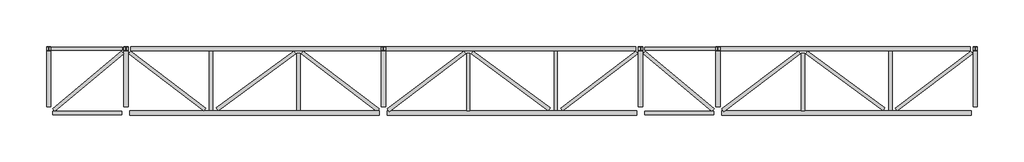
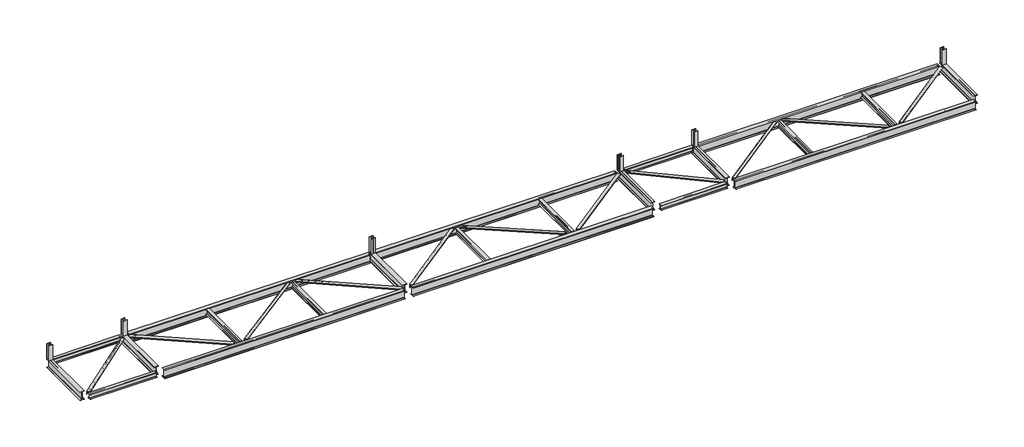
# One storey: 22 beams, 11 members, 6 columns.
"""IFC4 building model written with IfcOpenShell, lengths in millimetres."""

import ifcopenshell
import ifcopenshell.guid

model = None  # the IFC model being written
_history = None  # IfcOwnerHistory: only IFC2X3 demands one
_inside = {}  # id of a spatial element -> (the spatial element, [elements in it])
_under = {}  # id of a project, library or spatial element -> (it, [spatial elements below it])
_declared = {}  # id of a project -> (the project, [libraries it declares])
_typed = {}  # id of a type object -> (the type object, [elements of that type])
_made_of = {}  # id of a material, layer set ... -> (it, [elements and type objects made of it])


def new_model(schema):
    """Start an empty IFC model of exactly this schema.

    Asked for "IFC4X3", IfcOpenShell would pick the latest addendum, in which some entities
    have other attributes; the version numbers below select the first issue.
    IFC2X3 requires an IfcOwnerHistory on every rooted entity: one is made here for all.
    """
    global model, _history
    if schema == "IFC4X3":
        model = ifcopenshell.file(schema_version=(4, 3, 0, 0))
    else:
        model = ifcopenshell.file(schema=schema)
    _inside.clear()
    _under.clear()
    _declared.clear()
    _typed.clear()
    _made_of.clear()
    _history = None
    if model.schema == "IFC2X3":
        org = make("IfcOrganization", Name="unknown")
        user = make(
            "IfcPersonAndOrganization",
            ThePerson=make("IfcPerson", FamilyName="unknown"),
            TheOrganization=org,
        )
        app = make(
            "IfcApplication",
            ApplicationDeveloper=org,
            Version="unknown",
            ApplicationFullName="unknown",
            ApplicationIdentifier="unknown",
        )
        _history = make(
            "IfcOwnerHistory",
            OwningUser=user,
            OwningApplication=app,
            ChangeAction="ADDED",
            CreationDate=0,
        )
    return model


def make(cls, **values):
    """One entity of the class cls with the attributes given. An attribute that is None is left unset."""
    return model.create_entity(
        cls, **{name: value for name, value in values.items() if value is not None}
    )


def rooted(cls, **values):
    """An entity with a GlobalId (a new one), such as an element, a storey or a relation."""
    return make(cls, GlobalId=ifcopenshell.guid.new(), OwnerHistory=_history, **values)


def si_unit(unit_type, name, prefix=None):
    """IfcSIUnit, for example si_unit("LENGTHUNIT", "METRE", prefix="MILLI")."""
    return make("IfcSIUnit", UnitType=unit_type, Prefix=prefix, Name=name)


def assignment(units):
    """IfcUnitAssignment: the units of a project."""
    return None if units is None else make("IfcUnitAssignment", Units=units)


def point(xyz):
    """IfcCartesianPoint."""
    return None if xyz is None else make("IfcCartesianPoint", Coordinates=xyz)


def direction(xyz):
    """IfcDirection."""
    return None if xyz is None else make("IfcDirection", DirectionRatios=xyz)


def frame(location, z_axis=None, x_axis=None):
    """IfcAxis2Placement3D, a coordinate frame: its origin and axes. An axis left out is left unset."""
    return make(
        "IfcAxis2Placement3D",
        Location=point(location),
        Axis=direction(z_axis),
        RefDirection=direction(x_axis),
    )


def frame_2d(location, x_axis=None):
    """IfcAxis2Placement2D, a coordinate frame in the plane: its origin and x axis."""
    return make(
        "IfcAxis2Placement2D", Location=point(location), RefDirection=direction(x_axis)
    )


def origin():
    """The frame at (0, 0, 0) with its axes left unset."""
    return frame((0.0, 0.0, 0.0))


def place(relative_to, where):
    """IfcLocalPlacement: puts the frame where relative to a parent placement (None: the world)."""
    return make(
        "IfcLocalPlacement", PlacementRelTo=relative_to, RelativePlacement=where
    )


def context(
    kind, dimensions, precision=None, world=None, true_north=None, identifier=None
):
    """IfcGeometricRepresentationContext, for example the 3D "Model" context."""
    return make(
        "IfcGeometricRepresentationContext",
        ContextIdentifier=identifier,
        ContextType=kind,
        CoordinateSpaceDimension=dimensions,
        Precision=precision,
        WorldCoordinateSystem=world,
        TrueNorth=true_north,
    )


def project(units=None, contexts=None):
    """IfcProject with its units and contexts."""
    return rooted(
        "IfcProject",
        Name="project",
        RepresentationContexts=contexts,
        UnitsInContext=assignment(units),
    )


def spatial(cls, under=None, at=None, **own):
    """A site, building, storey or space (cls), placed at a placement, below another one or the project."""
    s = rooted(cls, ObjectPlacement=at, **own)
    if under is not None:
        _under.setdefault(under.id(), (under, []))[1].append(s)
    return s


def polyline(points):
    """IfcPolyline through the points."""
    return make("IfcPolyline", Points=[point(p) for p in points])


def circle_curve(where, radius):
    """IfcCircle in the frame where."""
    return make("IfcCircle", Position=where, Radius=radius)


def trimmed(basis, trim1, trim2, sense, master):
    """IfcTrimmedCurve: the piece of a basis curve between two trims."""
    return make(
        "IfcTrimmedCurve",
        BasisCurve=basis,
        Trim1=trim1,
        Trim2=trim2,
        SenseAgreement=sense,
        MasterRepresentation=master,
    )


def segment(curve, same_sense, transition):
    """IfcCompositeCurveSegment."""
    return make(
        "IfcCompositeCurveSegment",
        Transition=transition,
        SameSense=same_sense,
        ParentCurve=curve,
    )


def composite_curve(segments, self_intersect=None):
    """IfcCompositeCurve: segments joined end to end."""
    return make("IfcCompositeCurve", Segments=segments, SelfIntersect=self_intersect)


def outline(outer, holes=None, kind="AREA"):
    """IfcArbitraryClosedProfileDef: a profile drawn as a closed curve; with holes, ...WithVoids."""
    if holes is None:
        return make("IfcArbitraryClosedProfileDef", ProfileType=kind, OuterCurve=outer)
    return make(
        "IfcArbitraryProfileDefWithVoids",
        ProfileType=kind,
        OuterCurve=outer,
        InnerCurves=holes,
    )


def extrude(swept, where, along, depth):
    """IfcExtrudedAreaSolid: the profile swept, set in the frame where, extruded along a direction by depth."""
    return make(
        "IfcExtrudedAreaSolid",
        SweptArea=swept,
        Position=where,
        ExtrudedDirection=direction(along),
        Depth=depth,
    )


def shape(context_of_items, identifier, shape_type, items):
    """IfcShapeRepresentation: the items that make up one representation, for example the "Body"."""
    return make(
        "IfcShapeRepresentation",
        ContextOfItems=context_of_items,
        RepresentationIdentifier=identifier,
        RepresentationType=shape_type,
        Items=items,
    )


def source(mapping_origin, context_of_items, identifier, shape_type, items):
    """IfcRepresentationMap: a shape defined once, which mapped items show again and again."""
    return make(
        "IfcRepresentationMap",
        MappingOrigin=mapping_origin,
        MappedRepresentation=shape(context_of_items, identifier, shape_type, items),
    )


def transform(
    local_origin,
    x_axis=None,
    y_axis=None,
    z_axis=None,
    scale=None,
    scale2=None,
    scale3=None,
    uniform=True,
):
    """IfcCartesianTransformationOperator3D, or its non-uniform kind. x_axis, y_axis, z_axis: its Axis1, 2, 3."""
    if uniform:
        return make(
            "IfcCartesianTransformationOperator3D",
            Axis1=direction(x_axis),
            Axis2=direction(y_axis),
            LocalOrigin=point(local_origin),
            Scale=scale,
            Axis3=direction(z_axis),
        )
    return make(
        "IfcCartesianTransformationOperator3DnonUniform",
        Axis1=direction(x_axis),
        Axis2=direction(y_axis),
        LocalOrigin=point(local_origin),
        Scale=scale,
        Axis3=direction(z_axis),
        Scale2=scale2,
        Scale3=scale3,
    )


def mapped(mapping_source, mapping_target):
    """IfcMappedItem: shows the shape of a source again, moved by a transform."""
    return make(
        "IfcMappedItem", MappingSource=mapping_source, MappingTarget=mapping_target
    )


def made_of(thing, what):
    """Note that an element or type object is made of a material, layer set ...; save() writes the relation."""
    if what is not None:
        _made_of.setdefault(what.id(), (what, []))[1].append(thing)
    return thing


def element(
    cls,
    number,
    at=None,
    inside=None,
    cuts=None,
    type_object=None,
    material=None,
    context=None,
    identifier="Body",
    shape_type=None,
    held_by="IfcProductDefinitionShape",
    body=None,
    shapes=None,
    **own,
):
    """One element of the class cls, such as IfcWall. Its Tag is "e" and its number.

    at: its placement. inside: the storey or other place that contains it. cuts: it is an
    opening in that element (IfcRelVoidsElement). A single representation is given by context,
    identifier, shape_type and body (its items); several are given by shapes. held_by: the class
    of the entity that holds the representations. save() writes the other relations.
    """
    e = rooted(cls, Tag="e%d" % number, ObjectPlacement=at, **own)
    if body is not None:
        shapes = [shape(context, identifier, shape_type, body)]
    if shapes is not None:
        e.Representation = make(held_by, Representations=shapes)
    if inside is not None:
        _inside.setdefault(inside.id(), (inside, []))[1].append(e)
    if cuts is not None:
        rooted(
            "IfcRelVoidsElement", RelatingBuildingElement=cuts, RelatedOpeningElement=e
        )
    if type_object is not None:
        _typed.setdefault(type_object.id(), (type_object, []))[1].append(e)
    return made_of(e, material)


def aggregate(whole, parts):
    """IfcRelAggregates: a whole, such as a stair, and the parts it consists of."""
    return rooted("IfcRelAggregates", RelatingObject=whole, RelatedObjects=parts)


def save(model, path):
    """Write the relations noted so far, then the file.

    IfcRelAggregates (storeys below a building ...), IfcRelContainedInSpatialStructure (elements
    in a storey), IfcRelDefinesByType, IfcRelAssociatesMaterial and IfcRelDeclares: one each for
    every whole, place, type object, material and project.
    """
    for whole, parts in _under.values():
        aggregate(whole, parts)
    for where, things in _inside.values():
        rooted(
            "IfcRelContainedInSpatialStructure",
            RelatedElements=things,
            RelatingStructure=where,
        )
    for kind, things in _typed.values():
        rooted("IfcRelDefinesByType", RelatedObjects=things, RelatingType=kind)
    for what, things in _made_of.values():
        rooted("IfcRelAssociatesMaterial", RelatedObjects=things, RelatingMaterial=what)
    for by, libraries in _declared.values():
        rooted("IfcRelDeclares", RelatingContext=by, RelatedDefinitions=libraries)
    model.write(path)


def steel_framing_w_astm_a6m_f33feb28(model_context):
    return source(origin(), model_context, "Body", "SweptSolid", [
        extrude(outline(composite_curve([segment(polyline([(67.0, -94.8), (67.0, -105.0), (-67.0, -105.0), (-67.0, -94.8), (-10.775, -94.8)]), True, "CONTINUOUS"), segment(trimmed(circle_curve(frame_2d((-10.775, -87.2)), 7.6), [point((-10.775, -94.8))], [point((-3.175, -87.2))], True, "CARTESIAN"), True, "CONTINUOUS"), segment(polyline([(-3.175, -87.2), (-3.175, 87.2)]), True, "CONTINUOUS"), segment(trimmed(circle_curve(frame_2d((-10.775, 87.2)), 7.6), [point((-3.175, 87.2))], [point((-10.775, 94.8))], True, "CARTESIAN"), True, "CONTINUOUS"), segment(polyline([(-10.775, 94.8), (-67.0, 94.8), (-67.0, 105.0), (67.0, 105.0), (67.0, 94.8), (10.775, 94.8)]), True, "CONTINUOUS"), segment(trimmed(circle_curve(frame_2d((10.775, 87.2)), 7.6), [point((10.775, 94.8))], [point((3.175, 87.2))], True, "CARTESIAN"), True, "CONTINUOUS"), segment(polyline([(3.175, 87.2), (3.175, -87.2)]), True, "CONTINUOUS"), segment(trimmed(circle_curve(frame_2d((10.775, -87.2)), 7.6), [point((3.175, -87.2))], [point((10.775, -94.8))], True, "CARTESIAN"), True, "CONTINUOUS"), segment(polyline([(10.775, -94.8), (67.0, -94.8)]), True, "CONTINUOUS")], self_intersect=False)), frame((-1346.3, 0.0, 0.0), z_axis=(1.0, 0.0, 0.0), x_axis=(0.0, 1.0, 0.0)), (0.0, 0.0, 1.0), 2692.6),
    ])


def steel_framing_w_astm_a6m_aee8f6e1(model_context):
    return source(origin(), model_context, "Body", "SweptSolid", [
        extrude(outline(composite_curve([segment(polyline([(85.5, -166.4), (85.5, -178.0), (-85.5, -178.0), (-85.5, -166.4), (-13.72, -166.4)]), True, "CONTINUOUS"), segment(trimmed(circle_curve(frame_2d((-13.72, -156.3)), 10.1), [point((-13.72, -166.4))], [point((-3.62, -156.3))], True, "CARTESIAN"), True, "CONTINUOUS"), segment(polyline([(-3.62, -156.3), (-3.62, 156.3)]), True, "CONTINUOUS"), segment(trimmed(circle_curve(frame_2d((-13.72, 156.3)), 10.1), [point((-3.62, 156.3))], [point((-13.72, 166.4))], True, "CARTESIAN"), True, "CONTINUOUS"), segment(polyline([(-13.72, 166.4), (-85.5, 166.4), (-85.5, 178.0), (85.5, 178.0), (85.5, 166.4), (13.72, 166.4)]), True, "CONTINUOUS"), segment(trimmed(circle_curve(frame_2d((13.72, 156.3)), 10.1), [point((13.72, 166.4))], [point((3.62, 156.3))], True, "CARTESIAN"), True, "CONTINUOUS"), segment(polyline([(3.62, 156.3), (3.62, -156.3)]), True, "CONTINUOUS"), segment(trimmed(circle_curve(frame_2d((13.72, -156.3)), 10.1), [point((3.62, -156.3))], [point((13.72, -166.4))], True, "CARTESIAN"), True, "CONTINUOUS"), segment(polyline([(13.72, -166.4), (85.5, -166.4)]), True, "CONTINUOUS")], self_intersect=False)), frame((-4846.3, 0.0, 0.0), z_axis=(1.0, 0.0, 0.0), x_axis=(0.0, 1.0, 0.0)), (0.0, 0.0, 1.0), 9692.6),
    ])


def steel_framing_w_astm_a6m_761fb5d6(model_context):
    return source(origin(), model_context, "Body", "SweptSolid", [
        extrude(outline(composite_curve([segment(polyline([(85.5, -166.4), (85.5, -178.0), (-85.5, -178.0), (-85.5, -166.4), (-13.72, -166.4)]), True, "CONTINUOUS"), segment(trimmed(circle_curve(frame_2d((-13.72, -156.3)), 10.1), [point((-13.72, -166.4))], [point((-3.62, -156.3))], True, "CARTESIAN"), True, "CONTINUOUS"), segment(polyline([(-3.62, -156.3), (-3.62, 156.3)]), True, "CONTINUOUS"), segment(trimmed(circle_curve(frame_2d((-13.72, 156.3)), 10.1), [point((-3.62, 156.3))], [point((-13.72, 166.4))], True, "CARTESIAN"), True, "CONTINUOUS"), segment(polyline([(-13.72, 166.4), (-85.5, 166.4), (-85.5, 178.0), (85.5, 178.0), (85.5, 166.4), (13.72, 166.4)]), True, "CONTINUOUS"), segment(trimmed(circle_curve(frame_2d((13.72, 156.3)), 10.1), [point((13.72, 166.4))], [point((3.62, 156.3))], True, "CARTESIAN"), True, "CONTINUOUS"), segment(polyline([(3.62, 156.3), (3.62, -156.3)]), True, "CONTINUOUS"), segment(trimmed(circle_curve(frame_2d((13.72, -156.3)), 10.1), [point((3.62, -156.3))], [point((13.72, -166.4))], True, "CARTESIAN"), True, "CONTINUOUS"), segment(polyline([(13.72, -166.4), (85.5, -166.4)]), True, "CONTINUOUS")], self_intersect=False)), frame((-1003.8, 0.0, 0.0), z_axis=(1.0, 0.0, 0.0), x_axis=(0.0, 1.0, 0.0)), (0.0, 0.0, 1.0), 2339.3),
    ])


def steel_framing_w_astm_a6m_44bd27a9(model_context):
    return source(origin(), model_context, "Body", "SweptSolid", [
        extrude(outline(composite_curve([segment(polyline([(85.5, -166.4), (85.5, -178.0), (-85.5, -178.0), (-85.5, -166.4), (-13.72, -166.4)]), True, "CONTINUOUS"), segment(trimmed(circle_curve(frame_2d((-13.72, -156.3)), 10.1), [point((-13.72, -166.4))], [point((-3.62, -156.3))], True, "CARTESIAN"), True, "CONTINUOUS"), segment(polyline([(-3.62, -156.3), (-3.62, 156.3)]), True, "CONTINUOUS"), segment(trimmed(circle_curve(frame_2d((-13.72, 156.3)), 10.1), [point((-3.62, 156.3))], [point((-13.72, 166.4))], True, "CARTESIAN"), True, "CONTINUOUS"), segment(polyline([(-13.72, 166.4), (-85.5, 166.4), (-85.5, 178.0), (85.5, 178.0), (85.5, 166.4), (13.72, 166.4)]), True, "CONTINUOUS"), segment(trimmed(circle_curve(frame_2d((13.72, 156.3)), 10.1), [point((13.72, 166.4))], [point((3.62, 156.3))], True, "CARTESIAN"), True, "CONTINUOUS"), segment(polyline([(3.62, 156.3), (3.62, -156.3)]), True, "CONTINUOUS"), segment(trimmed(circle_curve(frame_2d((13.72, -156.3)), 10.1), [point((3.62, -156.3))], [point((13.72, -166.4))], True, "CARTESIAN"), True, "CONTINUOUS"), segment(polyline([(13.72, -166.4), (85.5, -166.4)]), True, "CONTINUOUS")], self_intersect=False)), frame((-1003.8, 0.0, 0.0), z_axis=(1.0, 0.0, 0.0), x_axis=(0.0, 1.0, 0.0)), (0.0, 0.0, 1.0), 2320.8),
    ])


def steel_framing_w_astm_a6m_88cf460a(model_context):
    return source(origin(), model_context, "Body", "SweptSolid", [
        extrude(outline(composite_curve([segment(polyline([(67.0, -94.8), (67.0, -105.0), (-67.0, -105.0), (-67.0, -94.8), (-10.775, -94.8)]), True, "CONTINUOUS"), segment(trimmed(circle_curve(frame_2d((-10.775, -87.2)), 7.6), [point((-10.775, -94.8))], [point((-3.175, -87.2))], True, "CARTESIAN"), True, "CONTINUOUS"), segment(polyline([(-3.175, -87.2), (-3.175, 87.2)]), True, "CONTINUOUS"), segment(trimmed(circle_curve(frame_2d((-10.775, 87.2)), 7.6), [point((-3.175, 87.2))], [point((-10.775, 94.8))], True, "CARTESIAN"), True, "CONTINUOUS"), segment(polyline([(-10.775, 94.8), (-67.0, 94.8), (-67.0, 105.0), (67.0, 105.0), (67.0, 94.8), (10.775, 94.8)]), True, "CONTINUOUS"), segment(trimmed(circle_curve(frame_2d((10.775, 87.2)), 7.6), [point((10.775, 94.8))], [point((3.175, 87.2))], True, "CARTESIAN"), True, "CONTINUOUS"), segment(polyline([(3.175, 87.2), (3.175, -87.2)]), True, "CONTINUOUS"), segment(trimmed(circle_curve(frame_2d((10.775, -87.2)), 7.6), [point((3.175, -87.2))], [point((10.775, -94.8))], True, "CARTESIAN"), True, "CONTINUOUS"), segment(polyline([(10.775, -94.8), (67.0, -94.8)]), True, "CONTINUOUS")], self_intersect=False)), frame((-1401.8, 0.0, 0.0), z_axis=(1.0, 0.0, 0.0), x_axis=(0.0, 1.0, 0.0)), (0.0, 0.0, 1.0), 2751.8),
    ])


def steel_framing_w_astm_a6m_bf6e2db3(model_context):
    return source(origin(), model_context, "Body", "SweptSolid", [
        extrude(outline(composite_curve([segment(polyline([(85.5, -166.4), (85.5, -178.0), (-85.5, -178.0), (-85.5, -166.4), (-13.72, -166.4)]), True, "CONTINUOUS"), segment(trimmed(circle_curve(frame_2d((-13.72, -156.3)), 10.1), [point((-13.72, -166.4))], [point((-3.62, -156.3))], True, "CARTESIAN"), True, "CONTINUOUS"), segment(polyline([(-3.62, -156.3), (-3.62, 156.3)]), True, "CONTINUOUS"), segment(trimmed(circle_curve(frame_2d((-13.72, 156.3)), 10.1), [point((-3.62, 156.3))], [point((-13.72, 166.4))], True, "CARTESIAN"), True, "CONTINUOUS"), segment(polyline([(-13.72, 166.4), (-85.5, 166.4), (-85.5, 178.0), (85.5, 178.0), (85.5, 166.4), (13.72, 166.4)]), True, "CONTINUOUS"), segment(trimmed(circle_curve(frame_2d((13.72, 156.3)), 10.1), [point((13.72, 166.4))], [point((3.62, 156.3))], True, "CARTESIAN"), True, "CONTINUOUS"), segment(polyline([(3.62, 156.3), (3.62, -156.3)]), True, "CONTINUOUS"), segment(trimmed(circle_curve(frame_2d((13.72, -156.3)), 10.1), [point((3.62, -156.3))], [point((13.72, -166.4))], True, "CARTESIAN"), True, "CONTINUOUS"), segment(polyline([(13.72, -166.4), (85.5, -166.4)]), True, "CONTINUOUS")], self_intersect=False)), frame((-4814.1, 0.0, 0.0), z_axis=(1.0, 0.0, 0.0), x_axis=(0.0, 1.0, 0.0)), (0.0, 0.0, 1.0), 9715.9),
    ])


def steel_framing_w_astm_a6m_6b735529(model_context):
    return source(origin(), model_context, "Body", "SweptSolid", [
        extrude(outline(composite_curve([segment(polyline([(67.0, -94.8), (67.0, -105.0), (-67.0, -105.0), (-67.0, -94.8), (-10.775, -94.8)]), True, "CONTINUOUS"), segment(trimmed(circle_curve(frame_2d((-10.775, -87.2)), 7.6), [point((-10.775, -94.8))], [point((-3.175, -87.2))], True, "CARTESIAN"), True, "CONTINUOUS"), segment(polyline([(-3.175, -87.2), (-3.175, 87.2)]), True, "CONTINUOUS"), segment(trimmed(circle_curve(frame_2d((-10.775, 87.2)), 7.6), [point((-3.175, 87.2))], [point((-10.775, 94.8))], True, "CARTESIAN"), True, "CONTINUOUS"), segment(polyline([(-10.775, 94.8), (-67.0, 94.8), (-67.0, 105.0), (67.0, 105.0), (67.0, 94.8), (10.775, 94.8)]), True, "CONTINUOUS"), segment(trimmed(circle_curve(frame_2d((10.775, 87.2)), 7.6), [point((10.775, 94.8))], [point((3.175, 87.2))], True, "CARTESIAN"), True, "CONTINUOUS"), segment(polyline([(3.175, 87.2), (3.175, -87.2)]), True, "CONTINUOUS"), segment(trimmed(circle_curve(frame_2d((10.775, -87.2)), 7.6), [point((3.175, -87.2))], [point((10.775, -94.8))], True, "CARTESIAN"), True, "CONTINUOUS"), segment(polyline([(10.775, -94.8), (67.0, -94.8)]), True, "CONTINUOUS")], self_intersect=False)), frame((-1140.8, 0.0, 0.0), z_axis=(1.0, 0.0, 0.0), x_axis=(0.0, 1.0, 0.0)), (0.0, 0.0, 1.0), 2292.6),
    ])


def steel_framing_w_astm_a6m_4302fd06(model_context):
    return source(origin(), model_context, "Body", "SweptSolid", [
        extrude(outline(composite_curve([segment(polyline([(67.0, -94.8), (67.0, -105.0), (-67.0, -105.0), (-67.0, -94.8), (-10.775, -94.8)]), True, "CONTINUOUS"), segment(trimmed(circle_curve(frame_2d((-10.775, -87.2)), 7.6), [point((-10.775, -94.8))], [point((-3.175, -87.2))], True, "CARTESIAN"), True, "CONTINUOUS"), segment(polyline([(-3.175, -87.2), (-3.175, 87.2)]), True, "CONTINUOUS"), segment(trimmed(circle_curve(frame_2d((-10.775, 87.2)), 7.6), [point((-3.175, 87.2))], [point((-10.775, 94.8))], True, "CARTESIAN"), True, "CONTINUOUS"), segment(polyline([(-10.775, 94.8), (-67.0, 94.8), (-67.0, 105.0), (67.0, 105.0), (67.0, 94.8), (10.775, 94.8)]), True, "CONTINUOUS"), segment(trimmed(circle_curve(frame_2d((10.775, 87.2)), 7.6), [point((10.775, 94.8))], [point((3.175, 87.2))], True, "CARTESIAN"), True, "CONTINUOUS"), segment(polyline([(3.175, 87.2), (3.175, -87.2)]), True, "CONTINUOUS"), segment(trimmed(circle_curve(frame_2d((10.775, -87.2)), 7.6), [point((3.175, -87.2))], [point((10.775, -94.8))], True, "CARTESIAN"), True, "CONTINUOUS"), segment(polyline([(10.775, -94.8), (67.0, -94.8)]), True, "CONTINUOUS")], self_intersect=False)), frame((-1151.8, 0.0, 0.0), z_axis=(1.0, 0.0, 0.0), x_axis=(0.0, 1.0, 0.0)), (0.0, 0.0, 1.0), 2220.9),
    ])


def steel_framing_w_astm_a6m_e8746ce3(model_context):
    return source(origin(), model_context, "Body", "SweptSolid", [
        extrude(outline(composite_curve([segment(polyline([(85.5, -166.4), (85.5, -178.0), (-85.5, -178.0), (-85.5, -166.4), (-13.72, -166.4)]), True, "CONTINUOUS"), segment(trimmed(circle_curve(frame_2d((-13.72, -156.3)), 10.1), [point((-13.72, -166.4))], [point((-3.62, -156.3))], True, "CARTESIAN"), True, "CONTINUOUS"), segment(polyline([(-3.62, -156.3), (-3.62, 156.3)]), True, "CONTINUOUS"), segment(trimmed(circle_curve(frame_2d((-13.72, 156.3)), 10.1), [point((-3.62, 156.3))], [point((-13.72, 166.4))], True, "CARTESIAN"), True, "CONTINUOUS"), segment(polyline([(-13.72, 166.4), (-85.5, 166.4), (-85.5, 178.0), (85.5, 178.0), (85.5, 166.4), (13.72, 166.4)]), True, "CONTINUOUS"), segment(trimmed(circle_curve(frame_2d((13.72, 156.3)), 10.1), [point((13.72, 166.4))], [point((3.62, 156.3))], True, "CARTESIAN"), True, "CONTINUOUS"), segment(polyline([(3.62, 156.3), (3.62, -156.3)]), True, "CONTINUOUS"), segment(trimmed(circle_curve(frame_2d((13.72, -156.3)), 10.1), [point((3.62, -156.3))], [point((13.72, -166.4))], True, "CARTESIAN"), True, "CONTINUOUS"), segment(polyline([(13.72, -166.4), (85.5, -166.4)]), True, "CONTINUOUS")], self_intersect=False)), frame((-4901.8, 0.0, 0.0), z_axis=(1.0, 0.0, 0.0), x_axis=(0.0, 1.0, 0.0)), (0.0, 0.0, 1.0), 9715.9),
    ])


def steel_framing_w_astm_a6m_fa6438b5(model_context):
    return source(origin(), model_context, "Body", "SweptSolid", [
        extrude(outline(composite_curve([segment(polyline([(67.0, -94.8), (67.0, -105.0), (-67.0, -105.0), (-67.0, -94.8), (-10.775, -94.8)]), True, "CONTINUOUS"), segment(trimmed(circle_curve(frame_2d((-10.775, -87.2)), 7.6), [point((-10.775, -94.8))], [point((-3.175, -87.2))], True, "CARTESIAN"), True, "CONTINUOUS"), segment(polyline([(-3.175, -87.2), (-3.175, 87.2)]), True, "CONTINUOUS"), segment(trimmed(circle_curve(frame_2d((-10.775, 87.2)), 7.6), [point((-3.175, 87.2))], [point((-10.775, 94.8))], True, "CARTESIAN"), True, "CONTINUOUS"), segment(polyline([(-10.775, 94.8), (-67.0, 94.8), (-67.0, 105.0), (67.0, 105.0), (67.0, 94.8), (10.775, 94.8)]), True, "CONTINUOUS"), segment(trimmed(circle_curve(frame_2d((10.775, 87.2)), 7.6), [point((10.775, 94.8))], [point((3.175, 87.2))], True, "CARTESIAN"), True, "CONTINUOUS"), segment(polyline([(3.175, 87.2), (3.175, -87.2)]), True, "CONTINUOUS"), segment(trimmed(circle_curve(frame_2d((10.775, -87.2)), 7.6), [point((3.175, -87.2))], [point((10.775, -94.8))], True, "CARTESIAN"), True, "CONTINUOUS"), segment(polyline([(10.775, -94.8), (67.0, -94.8)]), True, "CONTINUOUS")], self_intersect=False)), frame((-1350.0, 0.0, 0.0), z_axis=(1.0, 0.0, 0.0), x_axis=(0.0, 1.0, 0.0)), (0.0, 0.0, 1.0), 2751.8),
    ])


def steel_column_w_astm_a6m_853d7517(model_context):
    return source(origin(), model_context, "Body", "SweptSolid", [
        extrude(outline(composite_curve([segment(polyline([(76.5, 78.5), (76.5, 69.23), (9.63, 69.23)]), True, "CONTINUOUS"), segment(trimmed(circle_curve(frame_2d((9.63, 62.9)), 6.33), [point((9.63, 69.23))], [point((3.3, 62.9))], True, "CARTESIAN"), True, "CONTINUOUS"), segment(polyline([(3.3, 62.9), (3.3, -62.9)]), True, "CONTINUOUS"), segment(trimmed(circle_curve(frame_2d((9.63, -62.9)), 6.33), [point((3.3, -62.9))], [point((9.63, -69.23))], True, "CARTESIAN"), True, "CONTINUOUS"), segment(polyline([(9.63, -69.23), (76.5, -69.23), (76.5, -78.5), (-76.5, -78.5), (-76.5, -69.23), (-9.63, -69.23)]), True, "CONTINUOUS"), segment(trimmed(circle_curve(frame_2d((-9.63, -62.9)), 6.33), [point((-9.63, -69.23))], [point((-3.3, -62.9))], True, "CARTESIAN"), True, "CONTINUOUS"), segment(polyline([(-3.3, -62.9), (-3.3, 62.9)]), True, "CONTINUOUS"), segment(trimmed(circle_curve(frame_2d((-9.63, 62.9)), 6.33), [point((-3.3, 62.9))], [point((-9.63, 69.23))], True, "CARTESIAN"), True, "CONTINUOUS"), segment(polyline([(-9.63, 69.23), (-76.5, 69.23), (-76.5, 78.5), (76.5, 78.5)]), True, "CONTINUOUS")], self_intersect=False)), frame((0.0, 0.0, 1519.8243501), z_axis=(0.0, 0.0, 1.0), x_axis=(1.0, 0.0, 0.0)), (0.0, 0.0, 1.0), 644.0),
    ])


def member_96dd18ea(model_context):
    return source(origin(), model_context, "Body", "SweptSolid", [
        extrude(outline(composite_curve([segment(polyline([(36.4, 36.4), (36.4, -93.6)]), True, "CONTINUOUS"), segment(trimmed(circle_curve(frame_2d((36.4, -81.6)), 12.0), [point((36.4, -93.6))], [point((24.4, -81.6))], False, "CARTESIAN"), True, "CONTINUOUS"), segment(polyline([(24.4, -81.6), (24.4, 12.4)]), True, "CONTINUOUS"), segment(trimmed(circle_curve(frame_2d((12.4, 12.4)), 12.0), [point((24.4, 12.4))], [point((12.4, 24.4))], True, "CARTESIAN"), True, "CONTINUOUS"), segment(polyline([(12.4, 24.4), (-81.6, 24.4)]), True, "CONTINUOUS"), segment(trimmed(circle_curve(frame_2d((-81.6, 36.4)), 12.0), [point((-81.6, 24.4))], [point((-93.6, 36.4))], False, "CARTESIAN"), True, "CONTINUOUS"), segment(polyline([(-93.6, 36.4), (36.4, 36.4)]), True, "CONTINUOUS")], self_intersect=False)), frame((-1725.9882183, 0.0, 0.0), z_axis=(1.0, 0.0, 0.0), x_axis=(0.0, 1.0, 0.0)), (0.0, 0.0, 1.0), 3476.5545794),
    ])


def member_c24f28f7(model_context):
    return source(origin(), model_context, "Body", "SweptSolid", [
        extrude(outline(composite_curve([segment(polyline([(36.4, 36.4), (36.4, -93.6)]), True, "CONTINUOUS"), segment(trimmed(circle_curve(frame_2d((36.4, -81.6)), 12.0), [point((36.4, -93.6))], [point((24.4, -81.6))], False, "CARTESIAN"), True, "CONTINUOUS"), segment(polyline([(24.4, -81.6), (24.4, 12.4)]), True, "CONTINUOUS"), segment(trimmed(circle_curve(frame_2d((12.4, 12.4)), 12.0), [point((24.4, 12.4))], [point((12.4, 24.4))], True, "CARTESIAN"), True, "CONTINUOUS"), segment(polyline([(12.4, 24.4), (-81.6, 24.4)]), True, "CONTINUOUS"), segment(trimmed(circle_curve(frame_2d((-81.6, 36.4)), 12.0), [point((-81.6, 24.4))], [point((-93.6, 36.4))], False, "CARTESIAN"), True, "CONTINUOUS"), segment(polyline([(-93.6, 36.4), (36.4, 36.4)]), True, "CONTINUOUS")], self_intersect=False)), frame((-1867.6865023, 0.0, 0.0), z_axis=(1.0, 0.0, 0.0), x_axis=(0.0, 1.0, 0.0)), (0.0, 0.0, 1.0), 3659.8690046),
    ])


def member_3c30417d(model_context):
    return source(origin(), model_context, "Body", "SweptSolid", [
        extrude(outline(composite_curve([segment(polyline([(36.4, 36.4), (36.4, -93.6)]), True, "CONTINUOUS"), segment(trimmed(circle_curve(frame_2d((36.4, -81.6)), 12.0), [point((36.4, -93.6))], [point((24.4, -81.6))], False, "CARTESIAN"), True, "CONTINUOUS"), segment(polyline([(24.4, -81.6), (24.4, 12.4)]), True, "CONTINUOUS"), segment(trimmed(circle_curve(frame_2d((12.4, 12.4)), 12.0), [point((24.4, 12.4))], [point((12.4, 24.4))], True, "CARTESIAN"), True, "CONTINUOUS"), segment(polyline([(12.4, 24.4), (-81.6, 24.4)]), True, "CONTINUOUS"), segment(trimmed(circle_curve(frame_2d((-81.6, 36.4)), 12.0), [point((-81.6, 24.4))], [point((-93.6, 36.4))], False, "CARTESIAN"), True, "CONTINUOUS"), segment(polyline([(-93.6, 36.4), (36.4, 36.4)]), True, "CONTINUOUS")], self_intersect=False)), frame((-1825.7683013, 0.0, 0.0), z_axis=(1.0, 0.0, 0.0), x_axis=(0.0, 1.0, 0.0)), (0.0, 0.0, 1.0), 3729.3286027),
    ])


def member_c049ea03(model_context):
    return source(origin(), model_context, "Body", "SweptSolid", [
        extrude(outline(composite_curve([segment(polyline([(36.4, 36.4), (36.4, -93.6)]), True, "CONTINUOUS"), segment(trimmed(circle_curve(frame_2d((36.4, -81.6)), 12.0), [point((36.4, -93.6))], [point((24.4, -81.6))], False, "CARTESIAN"), True, "CONTINUOUS"), segment(polyline([(24.4, -81.6), (24.4, 12.4)]), True, "CONTINUOUS"), segment(trimmed(circle_curve(frame_2d((12.4, 12.4)), 12.0), [point((24.4, 12.4))], [point((12.4, 24.4))], True, "CARTESIAN"), True, "CONTINUOUS"), segment(polyline([(12.4, 24.4), (-81.6, 24.4)]), True, "CONTINUOUS"), segment(trimmed(circle_curve(frame_2d((-81.6, 36.4)), 12.0), [point((-81.6, 24.4))], [point((-93.6, 36.4))], False, "CARTESIAN"), True, "CONTINUOUS"), segment(polyline([(-93.6, 36.4), (36.4, 36.4)]), True, "CONTINUOUS")], self_intersect=False)), frame((-1867.6865023, 0.0, 0.0), z_axis=(1.0, 0.0, 0.0), x_axis=(0.0, 1.0, 0.0)), (0.0, 0.0, 1.0), 3720.541926),
    ])


def member_277812e4(model_context):
    return source(origin(), model_context, "Body", "SweptSolid", [
        extrude(outline(composite_curve([segment(polyline([(36.4, 36.4), (36.4, -93.6)]), True, "CONTINUOUS"), segment(trimmed(circle_curve(frame_2d((36.4, -81.6)), 12.0), [point((36.4, -93.6))], [point((24.4, -81.6))], False, "CARTESIAN"), True, "CONTINUOUS"), segment(polyline([(24.4, -81.6), (24.4, 12.4)]), True, "CONTINUOUS"), segment(trimmed(circle_curve(frame_2d((12.4, 12.4)), 12.0), [point((24.4, 12.4))], [point((12.4, 24.4))], True, "CARTESIAN"), True, "CONTINUOUS"), segment(polyline([(12.4, 24.4), (-81.6, 24.4)]), True, "CONTINUOUS"), segment(trimmed(circle_curve(frame_2d((-81.6, 36.4)), 12.0), [point((-81.6, 24.4))], [point((-93.6, 36.4))], False, "CARTESIAN"), True, "CONTINUOUS"), segment(polyline([(-93.6, 36.4), (36.4, 36.4)]), True, "CONTINUOUS")], self_intersect=False)), frame((-1852.8554237, 0.0, 0.0), z_axis=(1.0, 0.0, 0.0), x_axis=(0.0, 1.0, 0.0)), (0.0, 0.0, 1.0), 3720.541926),
    ])


def member_26543d8b(model_context):
    return source(origin(), model_context, "Body", "SweptSolid", [
        extrude(outline(composite_curve([segment(polyline([(36.4, 36.4), (36.4, -93.6)]), True, "CONTINUOUS"), segment(trimmed(circle_curve(frame_2d((36.4, -81.6)), 12.0), [point((36.4, -93.6))], [point((24.4, -81.6))], False, "CARTESIAN"), True, "CONTINUOUS"), segment(polyline([(24.4, -81.6), (24.4, 12.4)]), True, "CONTINUOUS"), segment(trimmed(circle_curve(frame_2d((12.4, 12.4)), 12.0), [point((24.4, 12.4))], [point((12.4, 24.4))], True, "CARTESIAN"), True, "CONTINUOUS"), segment(polyline([(12.4, 24.4), (-81.6, 24.4)]), True, "CONTINUOUS"), segment(trimmed(circle_curve(frame_2d((-81.6, 36.4)), 12.0), [point((-81.6, 24.4))], [point((-93.6, 36.4))], False, "CARTESIAN"), True, "CONTINUOUS"), segment(polyline([(-93.6, 36.4), (36.4, 36.4)]), True, "CONTINUOUS")], self_intersect=False)), frame((-1903.5603013, 0.0, 0.0), z_axis=(1.0, 0.0, 0.0), x_axis=(0.0, 1.0, 0.0)), (0.0, 0.0, 1.0), 3729.3286027),
    ])


def member_c6234845(model_context):
    return source(origin(), model_context, "Body", "SweptSolid", [
        extrude(outline(composite_curve([segment(polyline([(36.4, 36.4), (36.4, -93.6)]), True, "CONTINUOUS"), segment(trimmed(circle_curve(frame_2d((36.4, -81.6)), 12.0), [point((36.4, -93.6))], [point((24.4, -81.6))], False, "CARTESIAN"), True, "CONTINUOUS"), segment(polyline([(24.4, -81.6), (24.4, 12.4)]), True, "CONTINUOUS"), segment(trimmed(circle_curve(frame_2d((12.4, 12.4)), 12.0), [point((24.4, 12.4))], [point((12.4, 24.4))], True, "CARTESIAN"), True, "CONTINUOUS"), segment(polyline([(12.4, 24.4), (-81.6, 24.4)]), True, "CONTINUOUS"), segment(trimmed(circle_curve(frame_2d((-81.6, 36.4)), 12.0), [point((-81.6, 24.4))], [point((-93.6, 36.4))], False, "CARTESIAN"), True, "CONTINUOUS"), segment(polyline([(-93.6, 36.4), (36.4, 36.4)]), True, "CONTINUOUS")], self_intersect=False)), frame((-1792.1825023, 0.0, 0.0), z_axis=(1.0, 0.0, 0.0), x_axis=(0.0, 1.0, 0.0)), (0.0, 0.0, 1.0), 3659.8690046),
    ])


def member_46ab37a3(model_context):
    return source(origin(), model_context, "Body", "SweptSolid", [
        extrude(outline(composite_curve([segment(polyline([(36.4, 36.4), (36.4, -93.6)]), True, "CONTINUOUS"), segment(trimmed(circle_curve(frame_2d((36.4, -81.6)), 12.0), [point((36.4, -93.6))], [point((24.4, -81.6))], False, "CARTESIAN"), True, "CONTINUOUS"), segment(polyline([(24.4, -81.6), (24.4, 12.4)]), True, "CONTINUOUS"), segment(trimmed(circle_curve(frame_2d((12.4, 12.4)), 12.0), [point((24.4, 12.4))], [point((12.4, 24.4))], True, "CARTESIAN"), True, "CONTINUOUS"), segment(polyline([(12.4, 24.4), (-81.6, 24.4)]), True, "CONTINUOUS"), segment(trimmed(circle_curve(frame_2d((-81.6, 36.4)), 12.0), [point((-81.6, 24.4))], [point((-93.6, 36.4))], False, "CARTESIAN"), True, "CONTINUOUS"), segment(polyline([(-93.6, 36.4), (36.4, 36.4)]), True, "CONTINUOUS")], self_intersect=False)), frame((-1750.5663611, 0.0, 0.0), z_axis=(1.0, 0.0, 0.0), x_axis=(0.0, 1.0, 0.0)), (0.0, 0.0, 1.0), 3476.5545794),
    ])


model = new_model("IFC4")

# Units and contexts
model_context = context("Model", 3, world=origin())
ifc_project = project(units=[si_unit("LENGTHUNIT", "METRE", prefix="MILLI")], contexts=[model_context])

# Site, building, storey
site = spatial("IfcSite", under=ifc_project)
building = spatial("IfcBuilding", under=site)
storey = spatial("IfcBuildingStorey", under=building, Name="T.O.S(2-2)", Elevation=1519.8243501)

# Beams
placement = place(None, origin())
steel_framing_w_astm_a6m_shape = steel_framing_w_astm_a6m_f33feb28(model_context)
element("IfcBeam", 1, ObjectType="Steel Framing_W_ASTM A6M : H_SB_AR_S02_W200x31.3_B6", at=placement, inside=storey, context=model_context, shape_type="MappedRepresentation", body=[
    mapped(steel_framing_w_astm_a6m_shape, transform((1500.0, 14499.5208589, 1414.8243501), x_axis=(1.0, 0.0, 0.0), y_axis=(0.0, 1.0, 0.0), z_axis=(0.0, 0.0, 1.0))),
])
element("IfcBeam", 2, ObjectType="Steel Framing_W_ASTM A6M : H_SB_AR_S02_W200x31.3_B6", at=placement, inside=storey, context=model_context, shape_type="MappedRepresentation", body=[
    mapped(steel_framing_w_astm_a6m_shape, transform((24500.0, 14499.5208589, 1414.8243501), x_axis=(1.0, 0.0, 0.0), y_axis=(0.0, 1.0, 0.0), z_axis=(0.0, 0.0, 1.0))),
])
steel_framing_w_astm_a6m_2_shape = steel_framing_w_astm_a6m_aee8f6e1(model_context)
element("IfcBeam", 3, ObjectType="Steel Framing_W_ASTM A6M : H_SB_AR_S02_W360x51_B4", at=placement, inside=storey, context=model_context, shape_type="MappedRepresentation", body=[
    mapped(steel_framing_w_astm_a6m_2_shape, transform((8000.0, 14499.5208589, 1341.8243501), x_axis=(1.0, 0.0, 0.0), y_axis=(0.0, 1.0, 0.0), z_axis=(0.0, 0.0, 1.0))),
])
element("IfcBeam", 4, ObjectType="Steel Framing_W_ASTM A6M : H_SB_AR_S02_W360x51_B4", at=placement, inside=storey, context=model_context, shape_type="MappedRepresentation", body=[
    mapped(steel_framing_w_astm_a6m_2_shape, transform((18000.0, 14499.5208589, 1341.8243501), x_axis=(1.0, 0.0, 0.0), y_axis=(0.0, 1.0, 0.0), z_axis=(0.0, 0.0, 1.0))),
])
element("IfcBeam", 5, ObjectType="Steel Framing_W_ASTM A6M : H_SB_AR_S02_W360x51_B4", at=placement, inside=storey, context=model_context, shape_type="MappedRepresentation", body=[
    mapped(steel_framing_w_astm_a6m_2_shape, transform((31000.0, 14499.5208589, 1341.8243501), x_axis=(1.0, 0.0, 0.0), y_axis=(0.0, 1.0, 0.0), z_axis=(0.0, 0.0, 1.0))),
])
steel_framing_w_astm_a6m_3_shape = steel_framing_w_astm_a6m_761fb5d6(model_context)
element("IfcBeam", 6, ObjectType="Steel Framing_W_ASTM A6M : H_SB_AR_S02_W360x51_G3", at=placement, inside=storey, context=model_context, shape_type="MappedRepresentation", body=[
    mapped(steel_framing_w_astm_a6m_3_shape, transform((3000.0, 15749.5208589, 1341.8243501), x_axis=(0.0, 1.0, 0.0), y_axis=(-1.0, 0.0, 0.0), z_axis=(0.0, 0.0, 1.0))),
])
element("IfcBeam", 7, ObjectType="Steel Framing_W_ASTM A6M : H_SB_AR_S02_W360x51_G3", at=placement, inside=storey, context=model_context, shape_type="MappedRepresentation", body=[
    mapped(steel_framing_w_astm_a6m_3_shape, transform((13000.0, 15749.5208589, 1341.8243501), x_axis=(0.0, 1.0, 0.0), y_axis=(-1.0, 0.0, 0.0), z_axis=(0.0, 0.0, 1.0))),
])
element("IfcBeam", 8, ObjectType="Steel Framing_W_ASTM A6M : H_SB_AR_S02_W360x51_G3", at=placement, inside=storey, context=model_context, shape_type="MappedRepresentation", body=[
    mapped(steel_framing_w_astm_a6m_3_shape, transform((23000.0, 15749.5208589, 1341.8243501), x_axis=(0.0, 1.0, 0.0), y_axis=(-1.0, 0.0, 0.0), z_axis=(0.0, 0.0, 1.0))),
])
element("IfcBeam", 9, ObjectType="Steel Framing_W_ASTM A6M : H_SB_AR_S02_W360x51_G3", at=placement, inside=storey, context=model_context, shape_type="MappedRepresentation", body=[
    mapped(steel_framing_w_astm_a6m_3_shape, transform((26000.0, 15749.5208589, 1341.8243501), x_axis=(0.0, 1.0, 0.0), y_axis=(-1.0, 0.0, 0.0), z_axis=(0.0, 0.0, 1.0))),
])
element("IfcBeam", 10, ObjectType="Steel Framing_W_ASTM A6M : H_SB_AR_S02_W360x51_G3", at=placement, inside=storey, context=model_context, shape_type="MappedRepresentation", body=[
    mapped(steel_framing_w_astm_a6m_3_shape, transform((36000.0, 15749.5208589, 1341.8243501), x_axis=(0.0, 1.0, 0.0), y_axis=(-1.0, 0.0, 0.0), z_axis=(0.0, 0.0, 1.0))),
])
steel_framing_w_astm_a6m_4_shape = steel_framing_w_astm_a6m_44bd27a9(model_context)
element("IfcBeam", 11, ObjectType="Steel Framing_W_ASTM A6M : H_SB_AR_S02_W360x51_G3", at=placement, inside=storey, context=model_context, shape_type="MappedRepresentation", body=[
    mapped(steel_framing_w_astm_a6m_4_shape, transform((0.0, 15749.5208589, 1341.8243501), x_axis=(0.0, 1.0, 0.0), y_axis=(-1.0, 0.0, 0.0), z_axis=(0.0, 0.0, 1.0))),
])
steel_framing_w_astm_a6m_5_shape = steel_framing_w_astm_a6m_88cf460a(model_context)
element("IfcBeam", 12, ObjectType="Steel Framing_W_ASTM A6M : H_SB_AR_S02_W200x31.3_B6", at=placement, inside=storey, context=model_context, shape_type="MappedRepresentation", body=[
    mapped(steel_framing_w_astm_a6m_5_shape, transform((1500.0, 16999.5208589, 1414.8243501), x_axis=(1.0, 0.0, 0.0), y_axis=(0.0, 1.0, 0.0), z_axis=(0.0, 0.0, 1.0))),
])
steel_framing_w_astm_a6m_6_shape = steel_framing_w_astm_a6m_bf6e2db3(model_context)
element("IfcBeam", 13, ObjectType="Steel Framing_W_ASTM A6M : H_SB_AR_S02_W360x51_B4", at=placement, inside=storey, context=model_context, shape_type="MappedRepresentation", body=[
    mapped(steel_framing_w_astm_a6m_6_shape, transform((8000.0, 16999.5208589, 1341.8243501), x_axis=(1.0, 0.0, 0.0), y_axis=(0.0, 1.0, 0.0), z_axis=(0.0, 0.0, 1.0))),
])
steel_framing_w_astm_a6m_7_shape = steel_framing_w_astm_a6m_6b735529(model_context)
element("IfcBeam", 14, ObjectType="Steel Framing_W_ASTM A6M : H_SB_AR_S02_W200x31.3_B6", at=placement, inside=storey, context=model_context, shape_type="MappedRepresentation", body=[
    mapped(steel_framing_w_astm_a6m_7_shape, transform((6300.0, 15749.5208589, 1414.8243501), x_axis=(0.0, 1.0, 0.0), y_axis=(-1.0, 0.0, 0.0), z_axis=(0.0, 0.0, 1.0))),
])
element("IfcBeam", 15, ObjectType="Steel Framing_W_ASTM A6M : H_SB_AR_S02_W200x31.3_B6", at=placement, inside=storey, context=model_context, shape_type="MappedRepresentation", body=[
    mapped(steel_framing_w_astm_a6m_7_shape, transform((19700.0, 15749.5208589, 1414.8243501), x_axis=(0.0, 1.0, 0.0), y_axis=(-1.0, 0.0, 0.0), z_axis=(0.0, 0.0, 1.0))),
])
element("IfcBeam", 16, ObjectType="Steel Framing_W_ASTM A6M : H_SB_AR_S02_W200x31.3_B6", at=placement, inside=storey, context=model_context, shape_type="MappedRepresentation", body=[
    mapped(steel_framing_w_astm_a6m_7_shape, transform((32700.0, 15749.5208589, 1414.8243501), x_axis=(0.0, 1.0, 0.0), y_axis=(-1.0, 0.0, 0.0), z_axis=(0.0, 0.0, 1.0))),
])
steel_framing_w_astm_a6m_8_shape = steel_framing_w_astm_a6m_4302fd06(model_context)
element("IfcBeam", 17, ObjectType="Steel Framing_W_ASTM A6M : H_SB_AR_S02_W200x31.3_B6", at=placement, inside=storey, context=model_context, shape_type="MappedRepresentation", body=[
    mapped(steel_framing_w_astm_a6m_8_shape, transform((9700.0, 15749.5208589, 1414.8243501), x_axis=(0.0, 1.0, 0.0), y_axis=(-1.0, 0.0, 0.0), z_axis=(0.0, 0.0, 1.0))),
])
element("IfcBeam", 18, ObjectType="Steel Framing_W_ASTM A6M : H_SB_AR_S02_W200x31.3_B6", at=placement, inside=storey, context=model_context, shape_type="MappedRepresentation", body=[
    mapped(steel_framing_w_astm_a6m_8_shape, transform((16300.0, 15749.5208589, 1414.8243501), x_axis=(0.0, 1.0, 0.0), y_axis=(-1.0, 0.0, 0.0), z_axis=(0.0, 0.0, 1.0))),
])
element("IfcBeam", 19, ObjectType="Steel Framing_W_ASTM A6M : H_SB_AR_S02_W200x31.3_B6", at=placement, inside=storey, context=model_context, shape_type="MappedRepresentation", body=[
    mapped(steel_framing_w_astm_a6m_8_shape, transform((29300.0, 15749.5208589, 1414.8243501), x_axis=(0.0, 1.0, 0.0), y_axis=(-1.0, 0.0, 0.0), z_axis=(0.0, 0.0, 1.0))),
])
steel_framing_w_astm_a6m_9_shape = steel_framing_w_astm_a6m_e8746ce3(model_context)
element("IfcBeam", 20, ObjectType="Steel Framing_W_ASTM A6M : H_SB_AR_S02_W360x51_B4", at=placement, inside=storey, context=model_context, shape_type="MappedRepresentation", body=[
    mapped(steel_framing_w_astm_a6m_9_shape, transform((18000.0, 16999.5208589, 1341.8243501), x_axis=(1.0, 0.0, 0.0), y_axis=(0.0, 1.0, 0.0), z_axis=(0.0, 0.0, 1.0))),
])
element("IfcBeam", 21, ObjectType="Steel Framing_W_ASTM A6M : H_SB_AR_S02_W360x51_B4", at=placement, inside=storey, context=model_context, shape_type="MappedRepresentation", body=[
    mapped(steel_framing_w_astm_a6m_9_shape, transform((31000.0, 16999.5208589, 1341.8243501), x_axis=(1.0, 0.0, 0.0), y_axis=(0.0, 1.0, 0.0), z_axis=(0.0, 0.0, 1.0))),
])
steel_framing_w_astm_a6m_10_shape = steel_framing_w_astm_a6m_fa6438b5(model_context)
element("IfcBeam", 22, ObjectType="Steel Framing_W_ASTM A6M : H_SB_AR_S02_W200x31.3_B6", at=placement, inside=storey, context=model_context, shape_type="MappedRepresentation", body=[
    mapped(steel_framing_w_astm_a6m_10_shape, transform((24500.0, 16999.5208589, 1414.8243501), x_axis=(1.0, 0.0, 0.0), y_axis=(0.0, 1.0, 0.0), z_axis=(0.0, 0.0, 1.0))),
])

# Columns
steel_column_w_astm_a6m_shape = steel_column_w_astm_a6m_853d7517(model_context)
element("IfcColumn", 23, ObjectType="Steel Column_W_ASTM A6M : H_SC_AR_S01_W150x29.8_P1", at=placement, inside=storey, context=model_context, shape_type="MappedRepresentation", body=[
    mapped(steel_column_w_astm_a6m_shape, transform((0.0, 16999.5208589, 0.0), x_axis=(1.0, 0.0, 0.0), y_axis=(0.0, 1.0, 0.0), z_axis=(0.0, 0.0, 1.0))),
])
element("IfcColumn", 24, ObjectType="Steel Column_W_ASTM A6M : H_SC_AR_S01_W150x29.8_P1", at=placement, inside=storey, context=model_context, shape_type="MappedRepresentation", body=[
    mapped(steel_column_w_astm_a6m_shape, transform((3000.0, 16999.5208589, 0.0), x_axis=(1.0, 0.0, 0.0), y_axis=(0.0, 1.0, 0.0), z_axis=(0.0, 0.0, 1.0))),
])
element("IfcColumn", 25, ObjectType="Steel Column_W_ASTM A6M : H_SC_AR_S01_W150x29.8_P1", at=placement, inside=storey, context=model_context, shape_type="MappedRepresentation", body=[
    mapped(steel_column_w_astm_a6m_shape, transform((13000.0, 16999.5208589, 0.0), x_axis=(1.0, 0.0, 0.0), y_axis=(0.0, 1.0, 0.0), z_axis=(0.0, 0.0, 1.0))),
])
element("IfcColumn", 26, ObjectType="Steel Column_W_ASTM A6M : H_SC_AR_S01_W150x29.8_P1", at=placement, inside=storey, context=model_context, shape_type="MappedRepresentation", body=[
    mapped(steel_column_w_astm_a6m_shape, transform((26000.0, 16999.5208589, 0.0), x_axis=(1.0, 0.0, 0.0), y_axis=(0.0, 1.0, 0.0), z_axis=(0.0, 0.0, 1.0))),
])
element("IfcColumn", 27, ObjectType="Steel Column_W_ASTM A6M : H_SC_AR_S01_W150x29.8_P1", at=placement, inside=storey, context=model_context, shape_type="MappedRepresentation", body=[
    mapped(steel_column_w_astm_a6m_shape, transform((36000.0, 16999.5208589, 0.0), x_axis=(1.0, 0.0, 0.0), y_axis=(0.0, 1.0, 0.0), z_axis=(0.0, 0.0, 1.0))),
])
element("IfcColumn", 28, ObjectType="Steel Column_W_ASTM A6M : H_SC_AR_S01_W150x29.8_P2", at=placement, inside=storey, context=model_context, shape_type="MappedRepresentation", body=[
    mapped(steel_column_w_astm_a6m_shape, transform((23000.0, 16999.5208589, 0.0), x_axis=(1.0, 0.0, 0.0), y_axis=(0.0, 1.0, 0.0), z_axis=(0.0, 0.0, 1.0))),
])

# Members
member_shape = member_96dd18ea(model_context)
element("IfcMember", 29, ObjectType="0912_Steel Framing_L-KSD3502 : H_SB_AR_S03_L-130x130x12_HBR3", at=placement, inside=storey, context=model_context, shape_type="MappedRepresentation", body=[
    mapped(member_shape, transform((1500.0, 15749.5208589, 1483.4243501), x_axis=(0.768221279597377, 0.6401843996644785, 0.0), y_axis=(-0.6401843996644785, 0.768221279597377, 0.0), z_axis=(0.0, 0.0, 1.0))),
])
member_2_shape = member_c24f28f7(model_context)
element("IfcMember", 30, ObjectType="0912_Steel Framing_L-KSD3502 : H_SB_AR_S03_L-130x130x12_HBR3", at=placement, inside=storey, context=model_context, shape_type="MappedRepresentation", body=[
    mapped(member_2_shape, transform((4650.0, 15749.5208589, 1483.4243501), x_axis=(0.7970921481540102, -0.6038576879954627, 0.0), y_axis=(0.6038576879954627, 0.7970921481540102, 0.0), z_axis=(0.0, 0.0, 1.0))),
])
member_3_shape = member_3c30417d(model_context)
element("IfcMember", 31, ObjectType="0912_Steel Framing_L-KSD3502 : H_SB_AR_S03_L-130x130x12_HBR3", at=placement, inside=storey, context=model_context, shape_type="MappedRepresentation", body=[
    mapped(member_3_shape, transform((8000.0, 15749.5208589, 1483.4243501), x_axis=(0.8056510126494268, 0.5923904504775152, 0.0), y_axis=(-0.5923904504775152, 0.8056510126494268, 0.0), z_axis=(0.0, 0.0, 1.0))),
])
member_4_shape = member_c049ea03(model_context)
element("IfcMember", 32, ObjectType="0912_Steel Framing_L-KSD3502 : H_SB_AR_S03_L-130x130x12_HBR3", at=placement, inside=storey, context=model_context, shape_type="MappedRepresentation", body=[
    mapped(member_4_shape, transform((11350.0, 15749.5208589, 1483.4243501), x_axis=(0.7970921481540082, -0.6038576879954654, 0.0), y_axis=(0.6038576879954654, 0.7970921481540082, 0.0), z_axis=(0.0, 0.0, 1.0))),
])
member_5_shape = member_277812e4(model_context)
element("IfcMember", 33, ObjectType="0912_Steel Framing_L-KSD3502 : H_SB_AR_S03_L-130x130x12_HBR3", at=placement, inside=storey, context=model_context, shape_type="MappedRepresentation", body=[
    mapped(member_5_shape, transform((14650.0, 15749.5208589, 1483.4243501), x_axis=(0.7970921481540117, 0.6038576879954606, 0.0), y_axis=(-0.6038576879954606, 0.7970921481540117, 0.0), z_axis=(0.0, 0.0, 1.0))),
])
element("IfcMember", 34, ObjectType="0912_Steel Framing_L-KSD3502 : H_SB_AR_S03_L-130x130x12_HBR3", at=placement, inside=storey, context=model_context, shape_type="MappedRepresentation", body=[
    mapped(member_5_shape, transform((27650.0, 15749.5208589, 1483.4243501), x_axis=(0.7970921481540116, 0.6038576879954607, 0.0), y_axis=(-0.6038576879954607, 0.7970921481540116, 0.0), z_axis=(0.0, 0.0, 1.0))),
])
member_6_shape = member_26543d8b(model_context)
element("IfcMember", 35, ObjectType="0912_Steel Framing_L-KSD3502 : H_SB_AR_S03_L-130x130x12_HBR3", at=placement, inside=storey, context=model_context, shape_type="MappedRepresentation", body=[
    mapped(member_6_shape, transform((18000.0, 15749.5208589, 1483.4243501), x_axis=(0.8056510126494159, -0.5923904504775297, 0.0), y_axis=(0.5923904504775297, 0.8056510126494159, 0.0), z_axis=(0.0, 0.0, 1.0))),
])
element("IfcMember", 36, ObjectType="0912_Steel Framing_L-KSD3502 : H_SB_AR_S03_L-130x130x12_HBR3", at=placement, inside=storey, context=model_context, shape_type="MappedRepresentation", body=[
    mapped(member_6_shape, transform((31000.0, 15749.5208589, 1483.4243501), x_axis=(0.8056510126494139, -0.5923904504775325, 0.0), y_axis=(0.5923904504775325, 0.8056510126494139, 0.0), z_axis=(0.0, 0.0, 1.0))),
])
member_7_shape = member_c6234845(model_context)
element("IfcMember", 37, ObjectType="0912_Steel Framing_L-KSD3502 : H_SB_AR_S03_L-130x130x12_HBR3", at=placement, inside=storey, context=model_context, shape_type="MappedRepresentation", body=[
    mapped(member_7_shape, transform((21350.0, 15749.5208589, 1483.4243501), x_axis=(0.7970921481540116, 0.6038576879954607, 0.0), y_axis=(-0.6038576879954607, 0.7970921481540116, 0.0), z_axis=(0.0, 0.0, 1.0))),
])
element("IfcMember", 38, ObjectType="0912_Steel Framing_L-KSD3502 : H_SB_AR_S03_L-130x130x12_HBR3", at=placement, inside=storey, context=model_context, shape_type="MappedRepresentation", body=[
    mapped(member_7_shape, transform((34350.0, 15749.5208589, 1483.4243501), x_axis=(0.7970921481540116, 0.6038576879954608, 0.0), y_axis=(-0.6038576879954608, 0.7970921481540116, 0.0), z_axis=(0.0, 0.0, 1.0))),
])
member_8_shape = member_46ab37a3(model_context)
element("IfcMember", 39, ObjectType="0912_Steel Framing_L-KSD3502 : H_SB_AR_S03_L-130x130x12_HBR3", at=placement, inside=storey, context=model_context, shape_type="MappedRepresentation", body=[
    mapped(member_8_shape, transform((24500.0, 15749.5208589, 1483.4243501), x_axis=(0.7682212795973767, -0.6401843996644788, 0.0), y_axis=(0.6401843996644788, 0.7682212795973767, 0.0), z_axis=(0.0, 0.0, 1.0))),
])

save(model, "model.ifc")

# Revit data of these elements
# Type "Steel Framing_W_ASTM A6M : H_SB_AR_S02_W200x31.3_B6"
#   Type Mark = "B6"
#   Section Name Key = "W8x21"
#   Width = 13.4 cm
#   Web Thickness = 0.635 cm
#   Web Fillet = 0.76 cm
#   Warping Constant = 40800.0 cm⁶
#   Torsional Moment of Inertia = 11.70 cm⁴
#   Section Area = 39.7 cm²
#   Plastic Modulus weak axis = 93.2 cm³
#   Plastic Modulus strong axis = 334.0 cm³
#   Perimeter = 0.93 m²/m
#   Nominal Weight = 31.30 kgf/m
#   Moment of Inertia weak axis = 407.00 cm⁴
#   Moment of Inertia strong axis = 3130.00 cm⁴
#   Height = 21.0 cm
#   Flange Thickness = 1.02 cm
#   Elastic Modulus weak axis = 60.8 cm³
#   Elastic Modulus strong axis = 298.0 cm³
#   Centroid Vertical = 10.5 cm
#   Centroid Horizontal = 6.7 cm
#   Length [instance default] = 1500 mm
#   Structural Material [instance default] = Steel, 45-345
#   Bolt Spacing = 0
#   Assembly Code = ""
# Type "Steel Framing_W_ASTM A6M : H_SB_AR_S02_W360x51_B4"
#   Type Mark = "B4"
#   Section Name Key = "W14x34"
#   Width = 17.1 cm
#   Web Thickness = 0.724 cm
#   Web Fillet = 1.01 cm
#   Warping Constant = 287000.0 cm⁶
#   Torsional Moment of Inertia = 23.70 cm⁴
#   Section Area = 64.5 cm²
#   Plastic Modulus weak axis = 174.0 cm³
#   Plastic Modulus strong axis = 895.0 cm³
#   Perimeter = 1.36 m²/m
#   Nominal Weight = 51.00 kgf/m
#   Moment of Inertia weak axis = 970.00 cm⁴
#   Moment of Inertia strong axis = 14200.00 cm⁴
#   Height = 35.6 cm
#   Flange Thickness = 1.16 cm
#   Elastic Modulus weak axis = 113.0 cm³
#   Elastic Modulus strong axis = 796.0 cm³
#   Centroid Vertical = 17.8 cm
#   Centroid Horizontal = 8.55 cm
#   Length [instance default] = 1500 mm
#   Structural Material [instance default] = Steel, 45-345
#   Bolt Spacing = 0
#   Assembly Code = ""
# Type "Steel Framing_W_ASTM A6M : H_SB_AR_S02_W360x51_G3"
#   Type Mark = "G3"
#   Section Name Key = "W14x34"
#   Width = 17.1 cm
#   Web Thickness = 0.724 cm
#   Web Fillet = 1.01 cm
#   Warping Constant = 287000.0 cm⁶
#   Torsional Moment of Inertia = 23.70 cm⁴
#   Section Area = 64.5 cm²
#   Plastic Modulus weak axis = 174.0 cm³
#   Plastic Modulus strong axis = 895.0 cm³
#   Perimeter = 1.36 m²/m
#   Nominal Weight = 51.00 kgf/m
#   Moment of Inertia weak axis = 970.00 cm⁴
#   Moment of Inertia strong axis = 14200.00 cm⁴
#   Height = 35.6 cm
#   Flange Thickness = 1.16 cm
#   Elastic Modulus weak axis = 113.0 cm³
#   Elastic Modulus strong axis = 796.0 cm³
#   Centroid Vertical = 17.8 cm
#   Centroid Horizontal = 8.55 cm
#   Length [instance default] = 1500 mm
#   Structural Material [instance default] = Steel, 45-345
#   Bolt Spacing = 0
#   Assembly Code = ""
# Type "Steel Column_W_ASTM A6M : H_SC_AR_S01_W150x29.8_P1"
#   Section Name Key = "W6x20"
#   Width = 15.3 cm
#   Web Thickness = 0.66 cm
#   Web Fillet = 0.633 cm
#   Warping Constant = 30300.0 cm⁶
#   Torsional Moment of Inertia = 9.99 cm⁴
#   Section Area = 37.9 cm²
#   Plastic Modulus weak axis = 110.0 cm³
#   Plastic Modulus strong axis = 246.0 cm³
#   Perimeter = 0.902 m²/m
#   Nominal Weight = 29.80 kgf/m
#   Moment of Inertia weak axis = 554.00 cm⁴
#   Moment of Inertia strong axis = 1720.00 cm⁴
#   Height = 15.7 cm
#   Flange Thickness = 0.927 cm
#   Elastic Modulus weak axis = 72.3 cm³
#   Elastic Modulus strong axis = 220.0 cm³
#   Centroid Vertical = 7.85 cm
#   Centroid Horizontal = 7.65 cm
#   Structural Material [instance default] = Steel, 45-345
#   Bolt Spacing = 0
#   Assembly Code = ""
# Type "Steel Column_W_ASTM A6M : H_SC_AR_S01_W150x29.8_P2"
#   Section Name Key = "W6x20"
#   Width = 15.3 cm
#   Web Thickness = 0.66 cm
#   Web Fillet = 0.633 cm
#   Warping Constant = 30300.0 cm⁶
#   Torsional Moment of Inertia = 9.99 cm⁴
#   Section Area = 37.9 cm²
#   Plastic Modulus weak axis = 110.0 cm³
#   Plastic Modulus strong axis = 246.0 cm³
#   Perimeter = 0.902 m²/m
#   Nominal Weight = 29.80 kgf/m
#   Moment of Inertia weak axis = 554.00 cm⁴
#   Moment of Inertia strong axis = 1720.00 cm⁴
#   Height = 15.7 cm
#   Flange Thickness = 0.927 cm
#   Elastic Modulus weak axis = 72.3 cm³
#   Elastic Modulus strong axis = 220.0 cm³
#   Centroid Vertical = 7.85 cm
#   Centroid Horizontal = 7.65 cm
#   Structural Material [instance default] = Steel, 45-345
#   Bolt Spacing = 0
#   Assembly Code = ""
# Type "0912_Steel Framing_L-KSD3502 : H_SB_AR_S03_L-130x130x12_HBR3"
#   k = 25 mm
#   Perimeter = 0.52 m²/m
#   Nominal Weight = 23.40 kgf/m
#   Length [instance default] = 1000 mm
#   b = 130 mm
#   d = 130 mm
#   t = 12 mm
#   x = 36.4 mm
#   y = 36.4 mm
#   A = 2976.00 m²
#   Structural Material [instance default] = Steel, 45-345
# Elements 1, 2, 12, 14, 15, 16, 17, 18, 19, 22 (IfcBeam, "Steel Framing_W_ASTM A6M : H_SB_AR_S02_W200x31.3_B6")
#   Structural Material = Steel, 45-345
#   Phase Created = New Construction
#   Materials on its faces: "Steel, 45-345"
# Elements 3, 4, 5, 13, 20, 21 (IfcBeam, "Steel Framing_W_ASTM A6M : H_SB_AR_S02_W360x51_B4")
#   Structural Material = Steel, 45-345
#   Phase Created = New Construction
#   Materials on its faces: "Steel, 45-345"
# Elements 6, 7, 8, 9, 10, 11 (IfcBeam, "Steel Framing_W_ASTM A6M : H_SB_AR_S02_W360x51_G3")
#   Structural Material = Steel, 45-345
#   Phase Created = New Construction
#   Materials on its faces: "Steel, 45-345"
# Elements 23, 24, 25, 26, 27 (IfcColumn, "Steel Column_W_ASTM A6M : H_SC_AR_S01_W150x29.8_P1")
#   Comments = ""
#   Structural Material = Steel ASTM A992 GRADE 50
#   Phase Created = New Construction
#   Materials on its faces: "Steel ASTM A992 GRADE 50"
# Element 28 (IfcColumn, "Steel Column_W_ASTM A6M : H_SC_AR_S01_W150x29.8_P2")
#   Comments = ""
#   Structural Material = Steel ASTM A992 GRADE 50
#   Phase Created = New Construction
#   Materials on its faces: "Steel ASTM A992 GRADE 50"
# Elements 29, 30, 31, 32, 33, 34, 35, 36, 37, 38, 39 (IfcMember, "0912_Steel Framing_L-KSD3502 : H_SB_AR_S03_L-130x130x12_HBR3")
#   Structural Material = Steel ASTM A36
#   Phase Created = New Construction
#   Materials on its faces: "Steel ASTM A36"
# Materials
#   "Steel, 45-345": class "Metal", colour RGB 189 187 185, transparency 0, Description = "Steel 345 MPa", Cost = 0
#   "Steel ASTM A992 GRADE 50": class "Metal", colour RGB 120 120 120, transparency 0, Description = "Structural steel 50ksi", Cost = 0
#   "Steel ASTM A36": class "Metal", colour RGB 199 199 199, transparency 0, Description = "Structural steel, ASTM A36 Grade B, mill finish", Cost = 0
